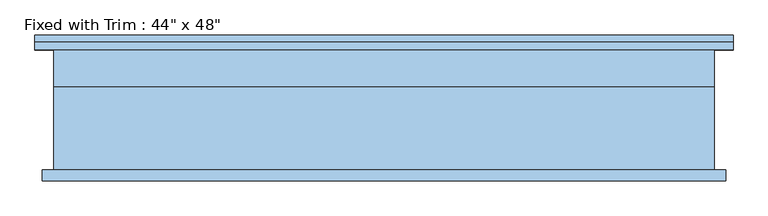
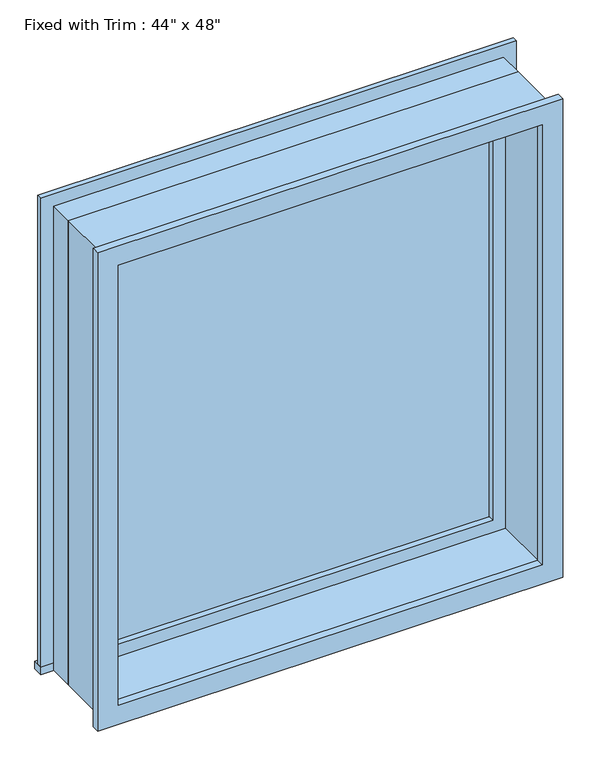
"""IFC4 building model written with IfcOpenShell, lengths in millimetres: window geometry."""

from ifc_helpers import new_model, si_unit, frame, origin, place, context, project, spatial, polyline, outline, extrude, source, transform, mapped, element, save


def window_db63b5d6(model_context):
    return source(origin(), model_context, "Body", "SweptSolid", [
        extrude(outline(polyline([(-628.65, 127.0), (552.45, 127.0), (552.45, 101.6), (-628.65, 101.6), (-628.65, 127.0)])), frame((0.0, 0.0, 914.4), z_axis=(0.0, 0.0, 1.0), x_axis=(1.0, 0.0, 0.0)), (0.0, 0.0, 1.0), 19.05),
        extrude(outline(polyline([(2114.55, -577.85), (2114.55, 501.65), (933.45, 501.65), (933.45, 552.45), (2165.35, 552.45), (2165.35, -628.65), (933.45, -628.65), (933.45, -577.85), (2114.55, -577.85)])), frame((0.0, 101.6, 0.0), z_axis=(0.0, 1.0, 0.0), x_axis=(0.0, 0.0, 1.0)), (0.0, 0.0, 1.0), 12.7),
        extrude(outline(polyline([(2152.65, 539.75), (2152.65, -615.95), (895.35, -615.95), (895.35, 539.75), (2152.65, 539.75)]), holes=[polyline([(2101.85, 488.95), (946.15, 488.95), (946.15, -565.15), (2101.85, -565.15), (2101.85, 488.95)])]), frame((0.0, -120.65, 0.0), z_axis=(0.0, 1.0, 0.0), x_axis=(0.0, 0.0, 1.0)), (0.0, 0.0, 1.0), 19.05),
        extrude(outline(polyline([(457.2, 53.975), (-533.4, 53.975), (-533.4, 66.675), (457.2, 66.675), (457.2, 53.975)])), frame((0.0, 0.0, 977.9), z_axis=(0.0, 0.0, 1.0), x_axis=(1.0, 0.0, 0.0)), (0.0, 0.0, 1.0), 1092.2),
        extrude(outline(polyline([(2114.55, -577.85), (933.45, -577.85), (933.45, 501.65), (2114.55, 501.65), (2114.55, -577.85)]), holes=[polyline([(2070.1, -533.4), (2070.1, 457.2), (977.9, 457.2), (977.9, -533.4), (2070.1, -533.4)])]), frame((0.0, 38.1, 0.0), z_axis=(0.0, 1.0, 0.0), x_axis=(0.0, 0.0, 1.0)), (0.0, 0.0, 1.0), 44.45),
        extrude(outline(polyline([(2133.6, -596.9), (914.4, -596.9), (914.4, 520.7), (2133.6, 520.7), (2133.6, -596.9)]), holes=[polyline([(2101.85, -565.15), (2101.85, 488.95), (946.15, 488.95), (946.15, -565.15), (2101.85, -565.15)])]), frame((0.0, -101.6, 0.0), z_axis=(0.0, 1.0, 0.0), x_axis=(0.0, 0.0, 1.0)), (0.0, 0.0, 1.0), 139.7),
        extrude(outline(polyline([(2133.6, 520.7), (2133.6, -596.9), (914.4, -596.9), (914.4, 520.7), (2133.6, 520.7)]), holes=[polyline([(2114.55, 501.65), (933.45, 501.65), (933.45, -577.85), (2114.55, -577.85), (2114.55, 501.65)])]), frame((0.0, 38.1, 0.0), z_axis=(0.0, 1.0, 0.0), x_axis=(0.0, 0.0, 1.0)), (0.0, 0.0, 1.0), 63.5),
    ])


if __name__ == "__main__":
    model = new_model("IFC4")
    model_context = context("Model", 3, world=origin())
    ifc_project = project(units=[si_unit("LENGTHUNIT", "METRE", prefix="MILLI")], contexts=[model_context])
    site = spatial("IfcSite", under=ifc_project)
    building = spatial("IfcBuilding", under=site)
    placement = place(None, origin())
    window_shape = window_db63b5d6(model_context)
    element("IfcWindow", 1, ObjectType="Fixed with Trim : 44\" x 48\"", at=placement, inside=building, context=model_context, shape_type="MappedRepresentation", body=[
        mapped(window_shape, transform((0.0, 0.0, 0.0), x_axis=(1.0, 0.0, 0.0), y_axis=(0.0, 1.0, 0.0), z_axis=(0.0, 0.0, 1.0))),
    ])
    save(model, "model.ifc")

# Revit data of these elements
# Type "Fixed with Trim : 44\" x 48\""
#   Type Mark = "89"
#   Assembly Code = "B2020100"
#   Height = 4' - 0"
#   Default Sill Height = 3' - 0"
#   Trim Projection - Ext. = 0' - 0 1/2"
#   Trim Projection - Int. = 0' - 0 3/4"
#   Trim Width - Exterior = 0' - 2"
#   Trim Width - Interior = 0' - 2"
#   Width = 3' - 8"
#   Window Inset = 0' - 0 3/4"
#   Glass Pane Material = Glass
#   Sash Material = Sash
#   Trim Exterior Material = Trim
#   Trim Interior Material = Trim
#   Wall Closure = (empty or 0)
# Element 1 (IfcWindow, "Fixed with Trim : 44\" x 48\"")
#   Materials on its faces: "Sash", "Trim", "Glass"
# Materials
#   "Glass": class "Glass", colour RGB 0 128 192, transparency 0.75
#   "Sash": class "Wood", colour RGB 224 178 126, transparency 0
#   "Trim": class "Wood", colour RGB 224 178 126, transparency 0
